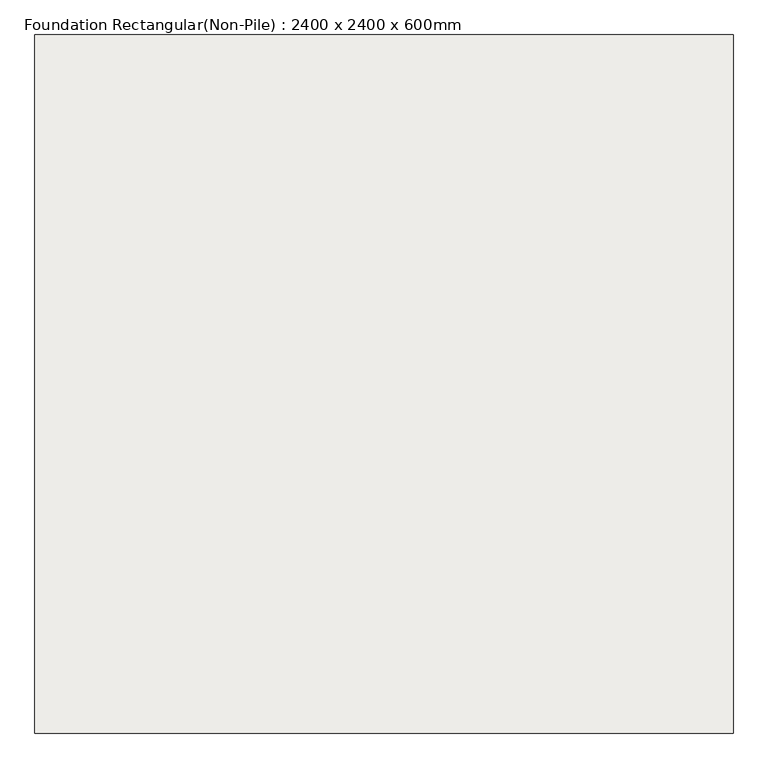
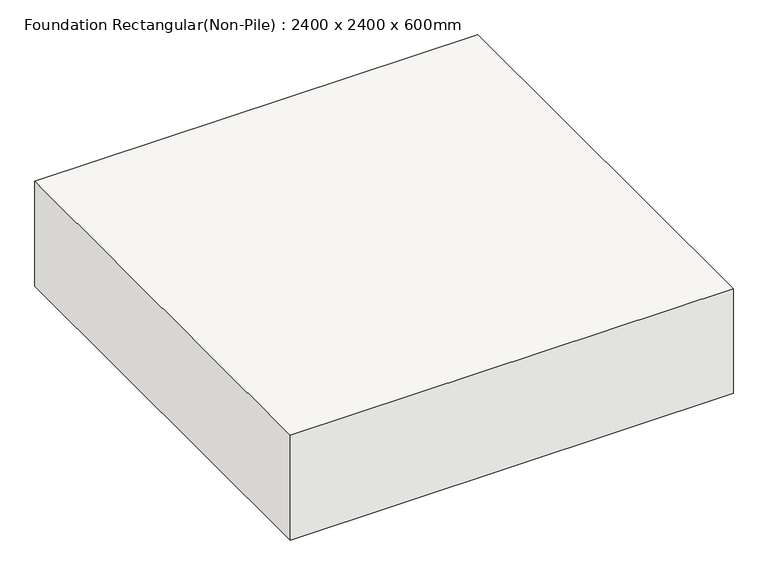
"""IFC4 building model written with IfcOpenShell, lengths in millimetres: slab geometry, Foundation Rectangular(Non-Pile) : 2400 x 2400 x 600mm."""

import ifcopenshell
import ifcopenshell.guid

model = None  # the IFC model being written
_history = None  # IfcOwnerHistory: only IFC2X3 demands one
_inside = {}  # id of a spatial element -> (the spatial element, [elements in it])
_under = {}  # id of a project, library or spatial element -> (it, [spatial elements below it])
_declared = {}  # id of a project -> (the project, [libraries it declares])
_typed = {}  # id of a type object -> (the type object, [elements of that type])
_made_of = {}  # id of a material, layer set ... -> (it, [elements and type objects made of it])


def new_model(schema):
    """Start an empty IFC model of exactly this schema.

    Asked for "IFC4X3", IfcOpenShell would pick the latest addendum, in which some entities
    have other attributes; the version numbers below select the first issue.
    IFC2X3 requires an IfcOwnerHistory on every rooted entity: one is made here for all.
    """
    global model, _history
    if schema == "IFC4X3":
        model = ifcopenshell.file(schema_version=(4, 3, 0, 0))
    else:
        model = ifcopenshell.file(schema=schema)
    _inside.clear()
    _under.clear()
    _declared.clear()
    _typed.clear()
    _made_of.clear()
    _history = None
    if model.schema == "IFC2X3":
        org = make("IfcOrganization", Name="unknown")
        user = make(
            "IfcPersonAndOrganization",
            ThePerson=make("IfcPerson", FamilyName="unknown"),
            TheOrganization=org,
        )
        app = make(
            "IfcApplication",
            ApplicationDeveloper=org,
            Version="unknown",
            ApplicationFullName="unknown",
            ApplicationIdentifier="unknown",
        )
        _history = make(
            "IfcOwnerHistory",
            OwningUser=user,
            OwningApplication=app,
            ChangeAction="ADDED",
            CreationDate=0,
        )
    return model


def make(cls, **values):
    """One entity of the class cls with the attributes given. An attribute that is None is left unset."""
    return model.create_entity(
        cls, **{name: value for name, value in values.items() if value is not None}
    )


def rooted(cls, **values):
    """An entity with a GlobalId (a new one), such as an element, a storey or a relation."""
    return make(cls, GlobalId=ifcopenshell.guid.new(), OwnerHistory=_history, **values)


def si_unit(unit_type, name, prefix=None):
    """IfcSIUnit, for example si_unit("LENGTHUNIT", "METRE", prefix="MILLI")."""
    return make("IfcSIUnit", UnitType=unit_type, Prefix=prefix, Name=name)


def assignment(units):
    """IfcUnitAssignment: the units of a project."""
    return None if units is None else make("IfcUnitAssignment", Units=units)


def point(xyz):
    """IfcCartesianPoint."""
    return None if xyz is None else make("IfcCartesianPoint", Coordinates=xyz)


def direction(xyz):
    """IfcDirection."""
    return None if xyz is None else make("IfcDirection", DirectionRatios=xyz)


def frame(location, z_axis=None, x_axis=None):
    """IfcAxis2Placement3D, a coordinate frame: its origin and axes. An axis left out is left unset."""
    return make(
        "IfcAxis2Placement3D",
        Location=point(location),
        Axis=direction(z_axis),
        RefDirection=direction(x_axis),
    )


def origin():
    """The frame at (0, 0, 0) with its axes left unset."""
    return frame((0.0, 0.0, 0.0))


def place(relative_to, where):
    """IfcLocalPlacement: puts the frame where relative to a parent placement (None: the world)."""
    return make(
        "IfcLocalPlacement", PlacementRelTo=relative_to, RelativePlacement=where
    )


def context(
    kind, dimensions, precision=None, world=None, true_north=None, identifier=None
):
    """IfcGeometricRepresentationContext, for example the 3D "Model" context."""
    return make(
        "IfcGeometricRepresentationContext",
        ContextIdentifier=identifier,
        ContextType=kind,
        CoordinateSpaceDimension=dimensions,
        Precision=precision,
        WorldCoordinateSystem=world,
        TrueNorth=true_north,
    )


def project(units=None, contexts=None):
    """IfcProject with its units and contexts."""
    return rooted(
        "IfcProject",
        Name="project",
        RepresentationContexts=contexts,
        UnitsInContext=assignment(units),
    )


def spatial(cls, under=None, at=None, **own):
    """A site, building, storey or space (cls), placed at a placement, below another one or the project."""
    s = rooted(cls, ObjectPlacement=at, **own)
    if under is not None:
        _under.setdefault(under.id(), (under, []))[1].append(s)
    return s


def polyline(points):
    """IfcPolyline through the points."""
    return make("IfcPolyline", Points=[point(p) for p in points])


def outline(outer, holes=None, kind="AREA"):
    """IfcArbitraryClosedProfileDef: a profile drawn as a closed curve; with holes, ...WithVoids."""
    if holes is None:
        return make("IfcArbitraryClosedProfileDef", ProfileType=kind, OuterCurve=outer)
    return make(
        "IfcArbitraryProfileDefWithVoids",
        ProfileType=kind,
        OuterCurve=outer,
        InnerCurves=holes,
    )


def extrude(swept, where, along, depth):
    """IfcExtrudedAreaSolid: the profile swept, set in the frame where, extruded along a direction by depth."""
    return make(
        "IfcExtrudedAreaSolid",
        SweptArea=swept,
        Position=where,
        ExtrudedDirection=direction(along),
        Depth=depth,
    )


def shape(context_of_items, identifier, shape_type, items):
    """IfcShapeRepresentation: the items that make up one representation, for example the "Body"."""
    return make(
        "IfcShapeRepresentation",
        ContextOfItems=context_of_items,
        RepresentationIdentifier=identifier,
        RepresentationType=shape_type,
        Items=items,
    )


def source(mapping_origin, context_of_items, identifier, shape_type, items):
    """IfcRepresentationMap: a shape defined once, which mapped items show again and again."""
    return make(
        "IfcRepresentationMap",
        MappingOrigin=mapping_origin,
        MappedRepresentation=shape(context_of_items, identifier, shape_type, items),
    )


def transform(
    local_origin,
    x_axis=None,
    y_axis=None,
    z_axis=None,
    scale=None,
    scale2=None,
    scale3=None,
    uniform=True,
):
    """IfcCartesianTransformationOperator3D, or its non-uniform kind. x_axis, y_axis, z_axis: its Axis1, 2, 3."""
    if uniform:
        return make(
            "IfcCartesianTransformationOperator3D",
            Axis1=direction(x_axis),
            Axis2=direction(y_axis),
            LocalOrigin=point(local_origin),
            Scale=scale,
            Axis3=direction(z_axis),
        )
    return make(
        "IfcCartesianTransformationOperator3DnonUniform",
        Axis1=direction(x_axis),
        Axis2=direction(y_axis),
        LocalOrigin=point(local_origin),
        Scale=scale,
        Axis3=direction(z_axis),
        Scale2=scale2,
        Scale3=scale3,
    )


def mapped(mapping_source, mapping_target):
    """IfcMappedItem: shows the shape of a source again, moved by a transform."""
    return make(
        "IfcMappedItem", MappingSource=mapping_source, MappingTarget=mapping_target
    )


def made_of(thing, what):
    """Note that an element or type object is made of a material, layer set ...; save() writes the relation."""
    if what is not None:
        _made_of.setdefault(what.id(), (what, []))[1].append(thing)
    return thing


def element(
    cls,
    number,
    at=None,
    inside=None,
    cuts=None,
    type_object=None,
    material=None,
    context=None,
    identifier="Body",
    shape_type=None,
    held_by="IfcProductDefinitionShape",
    body=None,
    shapes=None,
    **own,
):
    """One element of the class cls, such as IfcWall. Its Tag is "e" and its number.

    at: its placement. inside: the storey or other place that contains it. cuts: it is an
    opening in that element (IfcRelVoidsElement). A single representation is given by context,
    identifier, shape_type and body (its items); several are given by shapes. held_by: the class
    of the entity that holds the representations. save() writes the other relations.
    """
    e = rooted(cls, Tag="e%d" % number, ObjectPlacement=at, **own)
    if body is not None:
        shapes = [shape(context, identifier, shape_type, body)]
    if shapes is not None:
        e.Representation = make(held_by, Representations=shapes)
    if inside is not None:
        _inside.setdefault(inside.id(), (inside, []))[1].append(e)
    if cuts is not None:
        rooted(
            "IfcRelVoidsElement", RelatingBuildingElement=cuts, RelatedOpeningElement=e
        )
    if type_object is not None:
        _typed.setdefault(type_object.id(), (type_object, []))[1].append(e)
    return made_of(e, material)


def aggregate(whole, parts):
    """IfcRelAggregates: a whole, such as a stair, and the parts it consists of."""
    return rooted("IfcRelAggregates", RelatingObject=whole, RelatedObjects=parts)


def save(model, path):
    """Write the relations noted so far, then the file.

    IfcRelAggregates (storeys below a building ...), IfcRelContainedInSpatialStructure (elements
    in a storey), IfcRelDefinesByType, IfcRelAssociatesMaterial and IfcRelDeclares: one each for
    every whole, place, type object, material and project.
    """
    for whole, parts in _under.values():
        aggregate(whole, parts)
    for where, things in _inside.values():
        rooted(
            "IfcRelContainedInSpatialStructure",
            RelatedElements=things,
            RelatingStructure=where,
        )
    for kind, things in _typed.values():
        rooted("IfcRelDefinesByType", RelatedObjects=things, RelatingType=kind)
    for what, things in _made_of.values():
        rooted("IfcRelAssociatesMaterial", RelatedObjects=things, RelatingMaterial=what)
    for by, libraries in _declared.values():
        rooted("IfcRelDeclares", RelatingContext=by, RelatedDefinitions=libraries)
    model.write(path)


def foundation_rectangular_non_pile_2400_x_2400_x_600mm_9fdc1d6b(model_context):
    return source(origin(), model_context, "Body", "SweptSolid", [
        extrude(outline(polyline([(1200.0, 1200.0), (1200.0, -1200.0), (-1200.0, -1200.0), (-1200.0, 1200.0), (1200.0, 1200.0)])), frame((0.0, 0.0, -600.0), z_axis=(0.0, 0.0, 1.0), x_axis=(1.0, 0.0, 0.0)), (0.0, 0.0, 1.0), 600.0),
    ])


if __name__ == "__main__":
    model = new_model("IFC4")
    model_context = context("Model", 3, world=origin())
    ifc_project = project(units=[si_unit("LENGTHUNIT", "METRE", prefix="MILLI")], contexts=[model_context])
    site = spatial("IfcSite", under=ifc_project)
    building = spatial("IfcBuilding", under=site)
    placement = place(None, origin())
    foundation_rectangular_non_pile_2400_x_2400_x_600mm_shape = foundation_rectangular_non_pile_2400_x_2400_x_600mm_9fdc1d6b(model_context)
    element("IfcSlab", 1, ObjectType="Foundation Rectangular(Non-Pile) : 2400 x 2400 x 600mm", at=placement, inside=building, context=model_context, shape_type="MappedRepresentation", body=[
        mapped(foundation_rectangular_non_pile_2400_x_2400_x_600mm_shape, transform((0.0, 0.0, 0.0), x_axis=(1.0, 0.0, 0.0), y_axis=(0.0, 1.0, 0.0), z_axis=(0.0, 0.0, 1.0))),
    ])
    save(model, "model.ifc")

# Revit data of these elements
# Type "Foundation Rectangular(Non-Pile) : 2400 x 2400 x 600mm"
#   Width = 2400 mm
#   Length = 2400 mm
#   Foundation Thickness = 600 mm
#   Structural Material [instance default] = 콘크리트 - 현장타설 콘크리트
#   Assembly Code = ""
# Element 1 (IfcSlab, "Foundation Rectangular(Non-Pile) : 2400 x 2400 x 600mm")
#   Materials on its faces: "콘크리트 - 현장타설 콘크리트"
# Materials
#   "콘크리트 - 현장타설 콘크리트": class "콘크리트", colour RGB 192 192 192, transparency 0, Cost = 0
